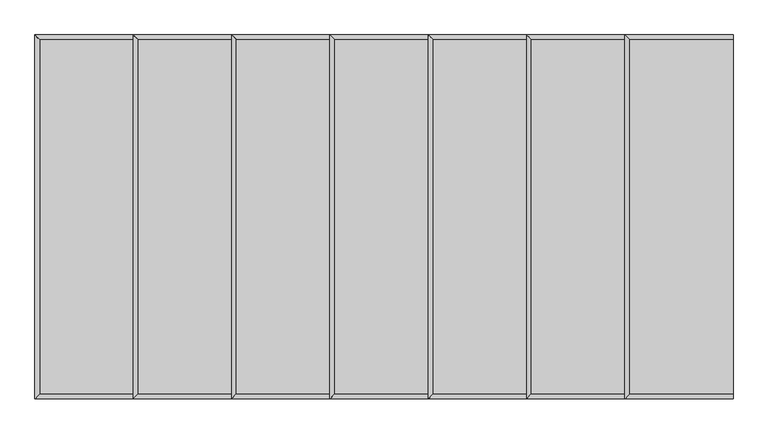
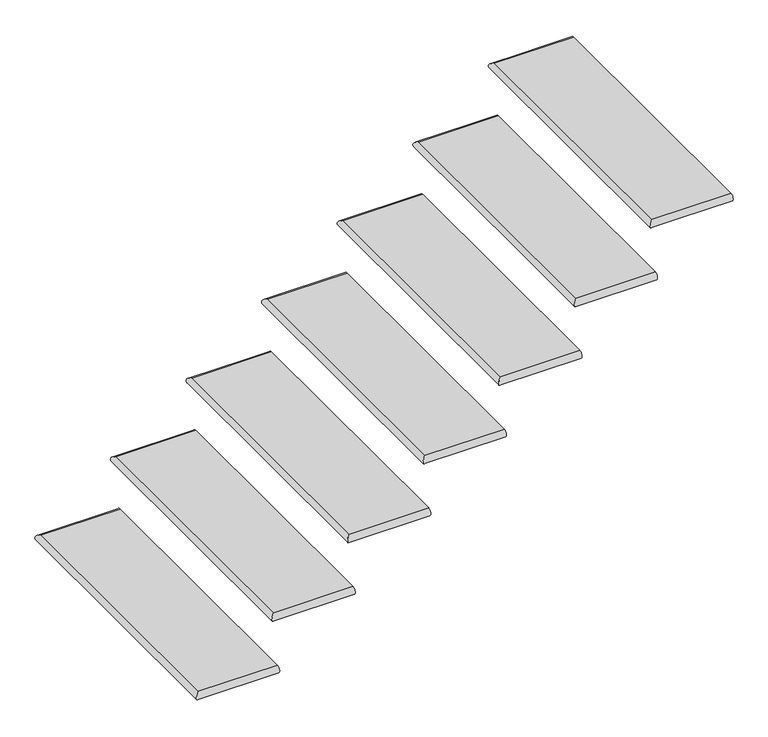
"""IFC4 building model written with IfcOpenShell, lengths in millimetres: stair flight geometry."""

from ifc_helpers import new_model, si_unit, frame, origin, place, context, project, spatial, circle_curve, ellipse_curve, source, transform, mapped, element, save
from ifc_brep_helpers import plane_surface, cylinder_surface, advanced_brep


def stair_flight_d73f07cf(model_context):
    return source(origin(), model_context, "Body", "AdvancedBrep", [
        advanced_brep(
        [(-17769.3481446, -11284.0871906, 165.1), (-17769.3481446, -11284.0871906, 190.5), (-17769.3481446, -10369.6871906, 190.5), (-17769.3481446, -10369.6871906, 165.1), (-17502.6481446, -11284.0871906, 190.5), (-17502.6481446, -10369.6871906, 190.5), (-17502.6481446, -10369.6871906, 165.1), (-17502.6481446, -11284.0871906, 165.1)],
        [
            (0, 1, ellipse_curve(frame((-17769.3481446, -11284.0871906, 177.8), z_axis=(-0.7071067811865465, 0.7071067811865487, 0.0), x_axis=(-0.7071067811865487, -0.7071067811865462, 0.0)), 17.9605122, 12.7)),
            (1, 2),
            (2, 3, ellipse_curve(frame((-17769.3481446, -10369.6871906, 177.8), z_axis=(-0.7071067811865486, -0.7071067811865464, 0.0), x_axis=(0.7071067811865464, -0.7071067811865488, 0.0)), 17.9605122, 12.7)),
            (3, 0),
            (4, 5),
            (5, 2),
            (1, 4),
            (6, 7),
            (7, 0),
            (3, 6),
            (4, 7, circle_curve(frame((-17502.6481446, -11284.0871906, 177.8), z_axis=(1.0, 0.0, 0.0), x_axis=(0.0, 1.0, 0.0)), 12.7)),
            (6, 5, circle_curve(frame((-17502.6481446, -10369.6871906, 177.8), z_axis=(1.0, 0.0, 0.0), x_axis=(0.0, -1.0, 0.0)), 12.7)),
        ],
        [
            cylinder_surface(frame((-17769.3481446, -11284.0871906, 177.8), z_axis=(0.0, -1.0, 0.0), x_axis=(1.0, 0.0, 0.0)), 12.7),
            plane_surface(frame((-17782.0481446, -10369.6871906, 190.5), z_axis=(0.0, 0.0, 1.0), x_axis=(-1.0, 0.0, 0.0))),
            plane_surface(frame((-17782.0481446, -10369.6871906, 165.1), z_axis=(0.0, 0.0, -1.0), x_axis=(1.0, 0.0, 0.0))),
            plane_surface(frame((-17502.6481446, -11284.0871906, 190.5), z_axis=(1.0, 0.0, 0.0), x_axis=(0.0, 0.0, -1.0))),
            cylinder_surface(frame((-17502.6481446, -11284.0871906, 177.8), z_axis=(1.0, 0.0, 0.0), x_axis=(0.0, 1.0, 0.0)), 12.7),
            cylinder_surface(frame((-17769.3481446, -10369.6871906, 177.8), z_axis=(-1.0, 0.0, 0.0), x_axis=(0.0, -1.0, 0.0)), 12.7),
        ],
        [
            (0, [[1, 2, 3, 4]]),
            (1, [[5, 6, -2, 7]]),
            (2, [[8, 9, -4, 10]]),
            (3, [[-5, 11, -8, 12]]),
            (4, [[-11, -7, -1, -9]]),
            (5, [[-3, -6, -12, -10]]),
        ],
    ),
        advanced_brep(
        [(-15978.6481446, -11284.0871906, 1333.5), (-15978.6481446, -10369.6871906, 1333.5), (-16245.3481446, -10369.6871906, 1333.5), (-16245.3481446, -11284.0871906, 1333.5), (-16004.0481446, -11284.0871906, 1333.5), (-15978.6481446, -10369.6871906, 1308.1), (-15978.6481446, -11284.0871906, 1308.1), (-16004.0481446, -11284.0871906, 1308.1), (-16245.3481446, -11284.0871906, 1308.1), (-16245.3481446, -10369.6871906, 1308.1)],
        [
            (0, 1),
            (1, 2),
            (2, 3),
            (3, 4),
            (4, 0),
            (5, 6),
            (6, 7),
            (7, 8),
            (8, 9),
            (9, 5),
            (0, 6, circle_curve(frame((-15978.6481446, -11284.0871906, 1320.8), z_axis=(1.0, 0.0, 0.0), x_axis=(0.0, 1.0, 0.0)), 12.7)),
            (5, 1, circle_curve(frame((-15978.6481446, -10369.6871906, 1320.8), z_axis=(1.0, 0.0, 0.0), x_axis=(0.0, -1.0, 0.0)), 12.7)),
            (8, 3, ellipse_curve(frame((-16245.3481446, -11284.0871906, 1320.8), z_axis=(-0.7071067811865475, 0.7071067811865475, 0.0), x_axis=(-0.7071067811865474, -0.7071067811865476, 0.0)), 17.9605122, 12.7)),
            (2, 9, ellipse_curve(frame((-16245.3481446, -10369.6871906, 1320.8), z_axis=(-0.7071067811865486, -0.7071067811865464, 0.0), x_axis=(0.7071067811865464, -0.7071067811865488, 0.0)), 17.9605122, 12.7)),
        ],
        [
            plane_surface(frame((-17782.0481446, -10369.6871906, 1333.5), z_axis=(0.0, 0.0, 1.0), x_axis=(-1.0, 0.0, 0.0))),
            plane_surface(frame((-17782.0481446, -10369.6871906, 1308.1), z_axis=(0.0, 0.0, -1.0), x_axis=(1.0, 0.0, 0.0))),
            plane_surface(frame((-15978.6481446, -11284.0871906, 1333.5), z_axis=(1.0, 0.0, 0.0), x_axis=(0.0, 0.0, -1.0))),
            cylinder_surface(frame((-16245.3481446, -11284.0871906, 1320.8), z_axis=(0.0, -1.0, 0.0), x_axis=(1.0, 0.0, 0.0)), 12.7),
            cylinder_surface(frame((-15978.6481446, -11284.0871906, 1320.8), z_axis=(1.0, 0.0, 0.0), x_axis=(0.0, 1.0, 0.0)), 12.7),
            cylinder_surface(frame((-16245.3481446, -10369.6871906, 1320.8), z_axis=(-1.0, 0.0, 0.0), x_axis=(0.0, -1.0, 0.0)), 12.7),
        ],
        [
            (0, [[1, 2, 3, 4, 5]]),
            (1, [[6, 7, 8, 9, 10]]),
            (2, [[-1, 11, -6, 12]]),
            (3, [[13, -3, 14, -9]]),
            (4, [[-11, -5, -4, -13, -8, -7]]),
            (5, [[-14, -2, -12, -10]]),
        ],
    ),
        advanced_brep(
        [(-17248.6481446, -11284.0871906, 381.0), (-17248.6481446, -10369.6871906, 381.0), (-17515.3481446, -10369.6871906, 381.0), (-17515.3481446, -11284.0871906, 381.0), (-17248.6481446, -10369.6871906, 355.6), (-17248.6481446, -11284.0871906, 355.6), (-17515.3481446, -11284.0871906, 355.6), (-17515.3481446, -10369.6871906, 355.6)],
        [
            (0, 1),
            (1, 2),
            (2, 3),
            (3, 0),
            (4, 5),
            (5, 6),
            (6, 7),
            (7, 4),
            (0, 5, circle_curve(frame((-17248.6481446, -11284.0871906, 368.3), z_axis=(1.0, 0.0, 0.0), x_axis=(0.0, 1.0, 0.0)), 12.7)),
            (4, 1, circle_curve(frame((-17248.6481446, -10369.6871906, 368.3), z_axis=(1.0, 0.0, 0.0), x_axis=(0.0, -1.0, 0.0)), 12.7)),
            (3, 6, ellipse_curve(frame((-17515.3481446, -11284.0871906, 368.3), z_axis=(0.7071067811865465, -0.7071067811865487, 0.0), x_axis=(0.7071067811865485, 0.7071067811865466, 0.0)), 17.9605122, 12.7)),
            (2, 7, ellipse_curve(frame((-17515.3481446, -10369.6871906, 368.3), z_axis=(-0.7071067811865486, -0.7071067811865464, 0.0), x_axis=(0.7071067811865464, -0.7071067811865488, 0.0)), 17.9605122, 12.7)),
        ],
        [
            plane_surface(frame((-17528.0481446, -10369.6871906, 381.0), z_axis=(0.0, 0.0, 1.0), x_axis=(-1.0, 0.0, 0.0))),
            plane_surface(frame((-17528.0481446, -10369.6871906, 355.6), z_axis=(0.0, 0.0, -1.0), x_axis=(1.0, 0.0, 0.0))),
            plane_surface(frame((-17248.6481446, -11284.0871906, 381.0), z_axis=(1.0, 0.0, 0.0), x_axis=(0.0, 0.0, -1.0))),
            cylinder_surface(frame((-17248.6481446, -11284.0871906, 368.3), z_axis=(1.0, 0.0, 0.0), x_axis=(0.0, 1.0, 0.0)), 12.7),
            cylinder_surface(frame((-17515.3481446, -11284.0871906, 368.3), z_axis=(0.0, -1.0, 0.0), x_axis=(1.0, 0.0, 0.0)), 12.7),
            cylinder_surface(frame((-17515.3481446, -10369.6871906, 368.3), z_axis=(-1.0, 0.0, 0.0), x_axis=(0.0, -1.0, 0.0)), 12.7),
        ],
        [
            (0, [[1, 2, 3, 4]]),
            (1, [[5, 6, 7, 8]]),
            (2, [[-1, 9, -5, 10]]),
            (3, [[-9, -4, 11, -6]]),
            (4, [[-11, -3, 12, -7]]),
            (5, [[-12, -2, -10, -8]]),
        ],
    ),
        advanced_brep(
        [(-16994.6481446, -11284.0871906, 571.5), (-16994.6481446, -10369.6871906, 571.5), (-17261.3481446, -10369.6871906, 571.5), (-17261.3481446, -11284.0871906, 571.5), (-16994.6481446, -10369.6871906, 546.1), (-16994.6481446, -11284.0871906, 546.1), (-17261.3481446, -11284.0871906, 546.1), (-17261.3481446, -10369.6871906, 546.1)],
        [
            (0, 1),
            (1, 2),
            (2, 3),
            (3, 0),
            (4, 5),
            (5, 6),
            (6, 7),
            (7, 4),
            (0, 5, circle_curve(frame((-16994.6481446, -11284.0871906, 558.8), z_axis=(1.0, 0.0, 0.0), x_axis=(0.0, 1.0, 0.0)), 12.7)),
            (4, 1, circle_curve(frame((-16994.6481446, -10369.6871906, 558.8), z_axis=(1.0, 0.0, 0.0), x_axis=(0.0, -1.0, 0.0)), 12.7)),
            (3, 6, ellipse_curve(frame((-17261.3481446, -11284.0871906, 558.8), z_axis=(0.7071067811865465, -0.7071067811865487, 0.0), x_axis=(0.7071067811865485, 0.7071067811865466, 0.0)), 17.9605122, 12.7)),
            (2, 7, ellipse_curve(frame((-17261.3481446, -10369.6871906, 558.8), z_axis=(-0.7071067811865486, -0.7071067811865464, 0.0), x_axis=(0.7071067811865464, -0.7071067811865488, 0.0)), 17.9605122, 12.7)),
        ],
        [
            plane_surface(frame((-17274.0481446, -10369.6871906, 571.5), z_axis=(0.0, 0.0, 1.0), x_axis=(-1.0, 0.0, 0.0))),
            plane_surface(frame((-17274.0481446, -10369.6871906, 546.1), z_axis=(0.0, 0.0, -1.0), x_axis=(1.0, 0.0, 0.0))),
            plane_surface(frame((-16994.6481446, -11284.0871906, 571.5), z_axis=(1.0, 0.0, 0.0), x_axis=(0.0, 0.0, -1.0))),
            cylinder_surface(frame((-16994.6481446, -11284.0871906, 558.8), z_axis=(1.0, 0.0, 0.0), x_axis=(0.0, 1.0, 0.0)), 12.7),
            cylinder_surface(frame((-17261.3481446, -11284.0871906, 558.8), z_axis=(0.0, -1.0, 0.0), x_axis=(1.0, 0.0, 0.0)), 12.7),
            cylinder_surface(frame((-17261.3481446, -10369.6871906, 558.8), z_axis=(-1.0, 0.0, 0.0), x_axis=(0.0, -1.0, 0.0)), 12.7),
        ],
        [
            (0, [[1, 2, 3, 4]]),
            (1, [[5, 6, 7, 8]]),
            (2, [[-1, 9, -5, 10]]),
            (3, [[-9, -4, 11, -6]]),
            (4, [[-11, -3, 12, -7]]),
            (5, [[-12, -2, -10, -8]]),
        ],
    ),
        advanced_brep(
        [(-16740.6481446, -11284.0871906, 762.0), (-16740.6481446, -10369.6871906, 762.0), (-17007.3481446, -10369.6871906, 762.0), (-17007.3481446, -11284.0871906, 762.0), (-16740.6481446, -10369.6871906, 736.6), (-16740.6481446, -11284.0871906, 736.6), (-17007.3481446, -11284.0871906, 736.6), (-17007.3481446, -10369.6871906, 736.6)],
        [
            (0, 1),
            (1, 2),
            (2, 3),
            (3, 0),
            (4, 5),
            (5, 6),
            (6, 7),
            (7, 4),
            (0, 5, circle_curve(frame((-16740.6481446, -11284.0871906, 749.3), z_axis=(1.0, 0.0, 0.0), x_axis=(0.0, 1.0, 0.0)), 12.7)),
            (4, 1, circle_curve(frame((-16740.6481446, -10369.6871906, 749.3), z_axis=(1.0, 0.0, 0.0), x_axis=(0.0, -1.0, 0.0)), 12.7)),
            (3, 6, ellipse_curve(frame((-17007.3481446, -11284.0871906, 749.3), z_axis=(0.7071067811865465, -0.7071067811865487, 0.0), x_axis=(0.7071067811865485, 0.7071067811865466, 0.0)), 17.9605122, 12.7)),
            (2, 7, ellipse_curve(frame((-17007.3481446, -10369.6871906, 749.3), z_axis=(-0.7071067811865486, -0.7071067811865464, 0.0), x_axis=(0.7071067811865464, -0.7071067811865488, 0.0)), 17.9605122, 12.7)),
        ],
        [
            plane_surface(frame((-17020.0481446, -10369.6871906, 762.0), z_axis=(0.0, 0.0, 1.0), x_axis=(-1.0, 0.0, 0.0))),
            plane_surface(frame((-17020.0481446, -10369.6871906, 736.6), z_axis=(0.0, 0.0, -1.0), x_axis=(1.0, 0.0, 0.0))),
            plane_surface(frame((-16740.6481446, -11284.0871906, 762.0), z_axis=(1.0, 0.0, 0.0), x_axis=(0.0, 0.0, -1.0))),
            cylinder_surface(frame((-16740.6481446, -11284.0871906, 749.3), z_axis=(1.0, 0.0, 0.0), x_axis=(0.0, 1.0, 0.0)), 12.7),
            cylinder_surface(frame((-17007.3481446, -11284.0871906, 749.3), z_axis=(0.0, -1.0, 0.0), x_axis=(1.0, 0.0, 0.0)), 12.7),
            cylinder_surface(frame((-17007.3481446, -10369.6871906, 749.3), z_axis=(-1.0, 0.0, 0.0), x_axis=(0.0, -1.0, 0.0)), 12.7),
        ],
        [
            (0, [[1, 2, 3, 4]]),
            (1, [[5, 6, 7, 8]]),
            (2, [[-1, 9, -5, 10]]),
            (3, [[-9, -4, 11, -6]]),
            (4, [[-11, -3, 12, -7]]),
            (5, [[-12, -2, -10, -8]]),
        ],
    ),
        advanced_brep(
        [(-16486.6481446, -11284.0871906, 952.5), (-16486.6481446, -10369.6871906, 952.5), (-16753.3481446, -10369.6871906, 952.5), (-16753.3481446, -11284.0871906, 952.5), (-16486.6481446, -10369.6871906, 927.1), (-16486.6481446, -11284.0871906, 927.1), (-16753.3481446, -11284.0871906, 927.1), (-16753.3481446, -10369.6871906, 927.1)],
        [
            (0, 1),
            (1, 2),
            (2, 3),
            (3, 0),
            (4, 5),
            (5, 6),
            (6, 7),
            (7, 4),
            (0, 5, circle_curve(frame((-16486.6481446, -11284.0871906, 939.8), z_axis=(1.0, 0.0, 0.0), x_axis=(0.0, 1.0, 0.0)), 12.7)),
            (4, 1, circle_curve(frame((-16486.6481446, -10369.6871906, 939.8), z_axis=(1.0, 0.0, 0.0), x_axis=(0.0, -1.0, 0.0)), 12.7)),
            (3, 6, ellipse_curve(frame((-16753.3481446, -11284.0871906, 939.8), z_axis=(0.7071067811865465, -0.7071067811865487, 0.0), x_axis=(0.7071067811865485, 0.7071067811865466, 0.0)), 17.9605122, 12.7)),
            (2, 7, ellipse_curve(frame((-16753.3481446, -10369.6871906, 939.8), z_axis=(-0.7071067811865486, -0.7071067811865464, 0.0), x_axis=(0.7071067811865464, -0.7071067811865488, 0.0)), 17.9605122, 12.7)),
        ],
        [
            plane_surface(frame((-16766.0481446, -10369.6871906, 952.5), z_axis=(0.0, 0.0, 1.0), x_axis=(-1.0, 0.0, 0.0))),
            plane_surface(frame((-16766.0481446, -10369.6871906, 927.1), z_axis=(0.0, 0.0, -1.0), x_axis=(1.0, 0.0, 0.0))),
            plane_surface(frame((-16486.6481446, -11284.0871906, 952.5), z_axis=(1.0, 0.0, 0.0), x_axis=(0.0, 0.0, -1.0))),
            cylinder_surface(frame((-16486.6481446, -11284.0871906, 939.8), z_axis=(1.0, 0.0, 0.0), x_axis=(0.0, 1.0, 0.0)), 12.7),
            cylinder_surface(frame((-16753.3481446, -11284.0871906, 939.8), z_axis=(0.0, -1.0, 0.0), x_axis=(1.0, 0.0, 0.0)), 12.7),
            cylinder_surface(frame((-16753.3481446, -10369.6871906, 939.8), z_axis=(-1.0, 0.0, 0.0), x_axis=(0.0, -1.0, 0.0)), 12.7),
        ],
        [
            (0, [[1, 2, 3, 4]]),
            (1, [[5, 6, 7, 8]]),
            (2, [[-1, 9, -5, 10]]),
            (3, [[-9, -4, 11, -6]]),
            (4, [[-11, -3, 12, -7]]),
            (5, [[-12, -2, -10, -8]]),
        ],
    ),
        advanced_brep(
        [(-16232.6481446, -11284.0871906, 1143.0), (-16232.6481446, -10369.6871906, 1143.0), (-16499.3481446, -10369.6871906, 1143.0), (-16499.3481446, -11284.0871906, 1143.0), (-16232.6481446, -10369.6871906, 1117.6), (-16232.6481446, -11284.0871906, 1117.6), (-16499.3481446, -11284.0871906, 1117.6), (-16499.3481446, -10369.6871906, 1117.6)],
        [
            (0, 1),
            (1, 2),
            (2, 3),
            (3, 0),
            (4, 5),
            (5, 6),
            (6, 7),
            (7, 4),
            (0, 5, circle_curve(frame((-16232.6481446, -11284.0871906, 1130.3), z_axis=(1.0, 0.0, 0.0), x_axis=(0.0, 1.0, 0.0)), 12.7)),
            (4, 1, circle_curve(frame((-16232.6481446, -10369.6871906, 1130.3), z_axis=(1.0, 0.0, 0.0), x_axis=(0.0, -1.0, 0.0)), 12.7)),
            (3, 6, ellipse_curve(frame((-16499.3481446, -11284.0871906, 1130.3), z_axis=(0.7071067811865465, -0.7071067811865487, 0.0), x_axis=(0.7071067811865485, 0.7071067811865466, 0.0)), 17.9605122, 12.7)),
            (2, 7, ellipse_curve(frame((-16499.3481446, -10369.6871906, 1130.3), z_axis=(-0.7071067811865486, -0.7071067811865464, 0.0), x_axis=(0.7071067811865464, -0.7071067811865488, 0.0)), 17.9605122, 12.7)),
        ],
        [
            plane_surface(frame((-16512.0481446, -10369.6871906, 1143.0), z_axis=(0.0, 0.0, 1.0), x_axis=(-1.0, 0.0, 0.0))),
            plane_surface(frame((-16512.0481446, -10369.6871906, 1117.6), z_axis=(0.0, 0.0, -1.0), x_axis=(1.0, 0.0, 0.0))),
            plane_surface(frame((-16232.6481446, -11284.0871906, 1143.0), z_axis=(1.0, 0.0, 0.0), x_axis=(0.0, 0.0, -1.0))),
            cylinder_surface(frame((-16232.6481446, -11284.0871906, 1130.3), z_axis=(1.0, 0.0, 0.0), x_axis=(0.0, 1.0, 0.0)), 12.7),
            cylinder_surface(frame((-16499.3481446, -11284.0871906, 1130.3), z_axis=(0.0, -1.0, 0.0), x_axis=(1.0, 0.0, 0.0)), 12.7),
            cylinder_surface(frame((-16499.3481446, -10369.6871906, 1130.3), z_axis=(-1.0, 0.0, 0.0), x_axis=(0.0, -1.0, 0.0)), 12.7),
        ],
        [
            (0, [[1, 2, 3, 4]]),
            (1, [[5, 6, 7, 8]]),
            (2, [[-1, 9, -5, 10]]),
            (3, [[-9, -4, 11, -6]]),
            (4, [[-11, -3, 12, -7]]),
            (5, [[-12, -2, -10, -8]]),
        ],
    ),
    ])


if __name__ == "__main__":
    model = new_model("IFC4")
    model_context = context("Model", 3, world=origin())
    ifc_project = project(units=[si_unit("LENGTHUNIT", "METRE", prefix="MILLI")], contexts=[model_context])
    site = spatial("IfcSite", under=ifc_project)
    building = spatial("IfcBuilding", under=site)
    placement = place(None, origin())
    stair_flight_shape = stair_flight_d73f07cf(model_context)
    element("IfcStairFlight", 1, at=placement, inside=building, context=model_context, shape_type="MappedRepresentation", body=[
        mapped(stair_flight_shape, transform((0.0, 0.0, 0.0), x_axis=(1.0, 0.0, 0.0), y_axis=(0.0, 1.0, 0.0), z_axis=(0.0, 0.0, 1.0))),
    ])
    save(model, "model.ifc")

# Revit data of these elements
# Element 1 (IfcStairFlight)
#   Materials on its faces: "Wood - Cherry"
# Materials
#   "Wood - Cherry": class "Unassigned", colour RGB 226 177 128, transparency 0
